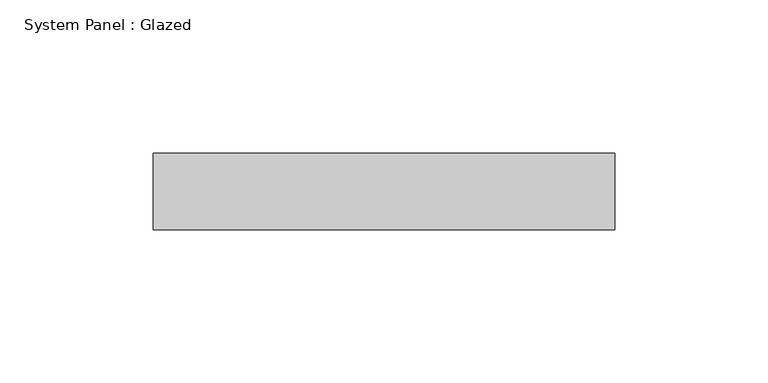
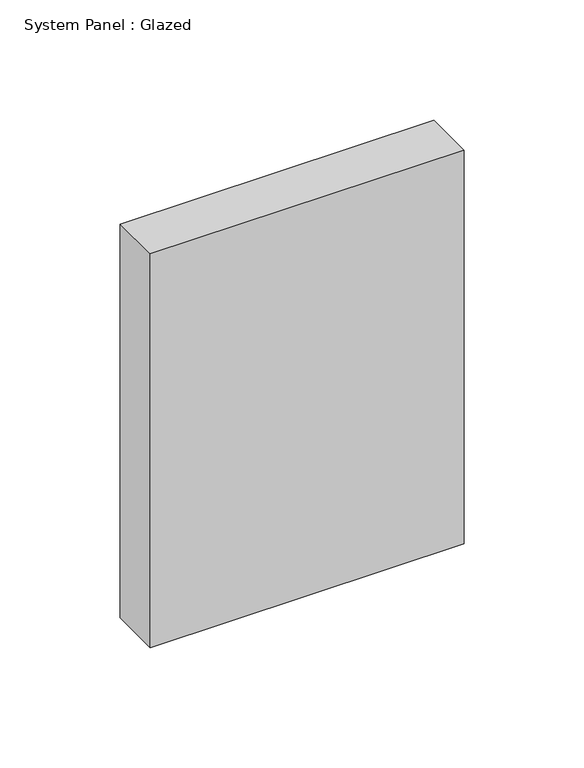
"""IFC4 building model written with IfcOpenShell, lengths in millimetres: plate geometry, System Panel : Glazed."""

from ifc_helpers import new_model, si_unit, origin, origin_with_axes, place, context, project, spatial, polyline, outline, extrude, source, transform, mapped, element, save


def system_panel_glazed_a3c9f580(model_context):
    return source(origin(), model_context, "Body", "SweptSolid", [
        extrude(outline(polyline([(75.3966098, 24.5), (-75.3966098, 24.5), (-75.3966098, 49.5), (75.3966098, 49.5), (75.3966098, 24.5)])), origin_with_axes(), (0.0, 0.0, 1.0), 200.0),
    ])


if __name__ == "__main__":
    model = new_model("IFC4")
    model_context = context("Model", 3, world=origin())
    ifc_project = project(units=[si_unit("LENGTHUNIT", "METRE", prefix="MILLI")], contexts=[model_context])
    site = spatial("IfcSite", under=ifc_project)
    building = spatial("IfcBuilding", under=site)
    placement = place(None, origin())
    system_panel_glazed_shape = system_panel_glazed_a3c9f580(model_context)
    element("IfcPlate", 1, ObjectType="System Panel : Glazed", at=placement, inside=building, context=model_context, shape_type="MappedRepresentation", body=[
        mapped(system_panel_glazed_shape, transform((0.0, 0.0, 0.0), x_axis=(1.0, 0.0, 0.0), y_axis=(0.0, 1.0, 0.0), z_axis=(0.0, 0.0, 1.0))),
    ])
    save(model, "model.ifc")

# Revit data of these elements
# Element 1 (IfcPlate, "System Panel : Glazed")
#   Materials on its faces: "Glass"
# Materials
#   "Glass": class "Glass", colour RGB 218 227 224, transparency 0.85, Description = "Soda Lime Glass", Cost = 0
